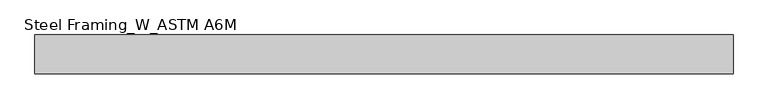
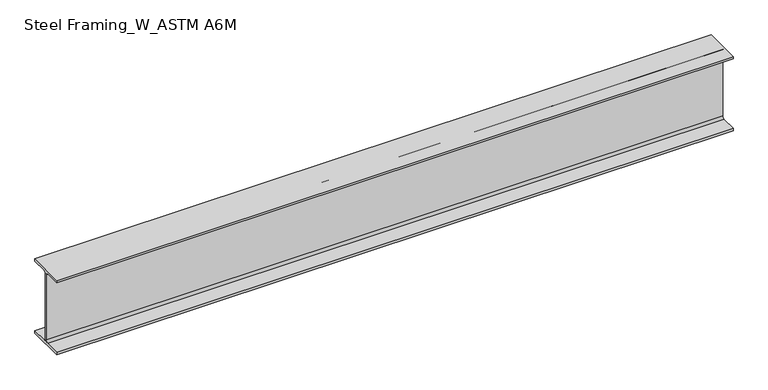
"""IFC4 building model written with IfcOpenShell, lengths in millimetres: beam geometry, Steel Framing_W_ASTM A6M : H_SB_AR_S02_W360x51_G3."""

import ifcopenshell
import ifcopenshell.guid

model = None  # the IFC model being written
_history = None  # IfcOwnerHistory: only IFC2X3 demands one
_inside = {}  # id of a spatial element -> (the spatial element, [elements in it])
_under = {}  # id of a project, library or spatial element -> (it, [spatial elements below it])
_declared = {}  # id of a project -> (the project, [libraries it declares])
_typed = {}  # id of a type object -> (the type object, [elements of that type])
_made_of = {}  # id of a material, layer set ... -> (it, [elements and type objects made of it])


def new_model(schema):
    """Start an empty IFC model of exactly this schema.

    Asked for "IFC4X3", IfcOpenShell would pick the latest addendum, in which some entities
    have other attributes; the version numbers below select the first issue.
    IFC2X3 requires an IfcOwnerHistory on every rooted entity: one is made here for all.
    """
    global model, _history
    if schema == "IFC4X3":
        model = ifcopenshell.file(schema_version=(4, 3, 0, 0))
    else:
        model = ifcopenshell.file(schema=schema)
    _inside.clear()
    _under.clear()
    _declared.clear()
    _typed.clear()
    _made_of.clear()
    _history = None
    if model.schema == "IFC2X3":
        org = make("IfcOrganization", Name="unknown")
        user = make(
            "IfcPersonAndOrganization",
            ThePerson=make("IfcPerson", FamilyName="unknown"),
            TheOrganization=org,
        )
        app = make(
            "IfcApplication",
            ApplicationDeveloper=org,
            Version="unknown",
            ApplicationFullName="unknown",
            ApplicationIdentifier="unknown",
        )
        _history = make(
            "IfcOwnerHistory",
            OwningUser=user,
            OwningApplication=app,
            ChangeAction="ADDED",
            CreationDate=0,
        )
    return model


def make(cls, **values):
    """One entity of the class cls with the attributes given. An attribute that is None is left unset."""
    return model.create_entity(
        cls, **{name: value for name, value in values.items() if value is not None}
    )


def rooted(cls, **values):
    """An entity with a GlobalId (a new one), such as an element, a storey or a relation."""
    return make(cls, GlobalId=ifcopenshell.guid.new(), OwnerHistory=_history, **values)


def si_unit(unit_type, name, prefix=None):
    """IfcSIUnit, for example si_unit("LENGTHUNIT", "METRE", prefix="MILLI")."""
    return make("IfcSIUnit", UnitType=unit_type, Prefix=prefix, Name=name)


def assignment(units):
    """IfcUnitAssignment: the units of a project."""
    return None if units is None else make("IfcUnitAssignment", Units=units)


def point(xyz):
    """IfcCartesianPoint."""
    return None if xyz is None else make("IfcCartesianPoint", Coordinates=xyz)


def direction(xyz):
    """IfcDirection."""
    return None if xyz is None else make("IfcDirection", DirectionRatios=xyz)


def frame(location, z_axis=None, x_axis=None):
    """IfcAxis2Placement3D, a coordinate frame: its origin and axes. An axis left out is left unset."""
    return make(
        "IfcAxis2Placement3D",
        Location=point(location),
        Axis=direction(z_axis),
        RefDirection=direction(x_axis),
    )


def frame_2d(location, x_axis=None):
    """IfcAxis2Placement2D, a coordinate frame in the plane: its origin and x axis."""
    return make(
        "IfcAxis2Placement2D", Location=point(location), RefDirection=direction(x_axis)
    )


def origin():
    """The frame at (0, 0, 0) with its axes left unset."""
    return frame((0.0, 0.0, 0.0))


def place(relative_to, where):
    """IfcLocalPlacement: puts the frame where relative to a parent placement (None: the world)."""
    return make(
        "IfcLocalPlacement", PlacementRelTo=relative_to, RelativePlacement=where
    )


def context(
    kind, dimensions, precision=None, world=None, true_north=None, identifier=None
):
    """IfcGeometricRepresentationContext, for example the 3D "Model" context."""
    return make(
        "IfcGeometricRepresentationContext",
        ContextIdentifier=identifier,
        ContextType=kind,
        CoordinateSpaceDimension=dimensions,
        Precision=precision,
        WorldCoordinateSystem=world,
        TrueNorth=true_north,
    )


def project(units=None, contexts=None):
    """IfcProject with its units and contexts."""
    return rooted(
        "IfcProject",
        Name="project",
        RepresentationContexts=contexts,
        UnitsInContext=assignment(units),
    )


def spatial(cls, under=None, at=None, **own):
    """A site, building, storey or space (cls), placed at a placement, below another one or the project."""
    s = rooted(cls, ObjectPlacement=at, **own)
    if under is not None:
        _under.setdefault(under.id(), (under, []))[1].append(s)
    return s


def polyline(points):
    """IfcPolyline through the points."""
    return make("IfcPolyline", Points=[point(p) for p in points])


def circle_curve(where, radius):
    """IfcCircle in the frame where."""
    return make("IfcCircle", Position=where, Radius=radius)


def trimmed(basis, trim1, trim2, sense, master):
    """IfcTrimmedCurve: the piece of a basis curve between two trims."""
    return make(
        "IfcTrimmedCurve",
        BasisCurve=basis,
        Trim1=trim1,
        Trim2=trim2,
        SenseAgreement=sense,
        MasterRepresentation=master,
    )


def segment(curve, same_sense, transition):
    """IfcCompositeCurveSegment."""
    return make(
        "IfcCompositeCurveSegment",
        Transition=transition,
        SameSense=same_sense,
        ParentCurve=curve,
    )


def composite_curve(segments, self_intersect=None):
    """IfcCompositeCurve: segments joined end to end."""
    return make("IfcCompositeCurve", Segments=segments, SelfIntersect=self_intersect)


def outline(outer, holes=None, kind="AREA"):
    """IfcArbitraryClosedProfileDef: a profile drawn as a closed curve; with holes, ...WithVoids."""
    if holes is None:
        return make("IfcArbitraryClosedProfileDef", ProfileType=kind, OuterCurve=outer)
    return make(
        "IfcArbitraryProfileDefWithVoids",
        ProfileType=kind,
        OuterCurve=outer,
        InnerCurves=holes,
    )


def extrude(swept, where, along, depth):
    """IfcExtrudedAreaSolid: the profile swept, set in the frame where, extruded along a direction by depth."""
    return make(
        "IfcExtrudedAreaSolid",
        SweptArea=swept,
        Position=where,
        ExtrudedDirection=direction(along),
        Depth=depth,
    )


def shape(context_of_items, identifier, shape_type, items):
    """IfcShapeRepresentation: the items that make up one representation, for example the "Body"."""
    return make(
        "IfcShapeRepresentation",
        ContextOfItems=context_of_items,
        RepresentationIdentifier=identifier,
        RepresentationType=shape_type,
        Items=items,
    )


def source(mapping_origin, context_of_items, identifier, shape_type, items):
    """IfcRepresentationMap: a shape defined once, which mapped items show again and again."""
    return make(
        "IfcRepresentationMap",
        MappingOrigin=mapping_origin,
        MappedRepresentation=shape(context_of_items, identifier, shape_type, items),
    )


def transform(
    local_origin,
    x_axis=None,
    y_axis=None,
    z_axis=None,
    scale=None,
    scale2=None,
    scale3=None,
    uniform=True,
):
    """IfcCartesianTransformationOperator3D, or its non-uniform kind. x_axis, y_axis, z_axis: its Axis1, 2, 3."""
    if uniform:
        return make(
            "IfcCartesianTransformationOperator3D",
            Axis1=direction(x_axis),
            Axis2=direction(y_axis),
            LocalOrigin=point(local_origin),
            Scale=scale,
            Axis3=direction(z_axis),
        )
    return make(
        "IfcCartesianTransformationOperator3DnonUniform",
        Axis1=direction(x_axis),
        Axis2=direction(y_axis),
        LocalOrigin=point(local_origin),
        Scale=scale,
        Axis3=direction(z_axis),
        Scale2=scale2,
        Scale3=scale3,
    )


def mapped(mapping_source, mapping_target):
    """IfcMappedItem: shows the shape of a source again, moved by a transform."""
    return make(
        "IfcMappedItem", MappingSource=mapping_source, MappingTarget=mapping_target
    )


def made_of(thing, what):
    """Note that an element or type object is made of a material, layer set ...; save() writes the relation."""
    if what is not None:
        _made_of.setdefault(what.id(), (what, []))[1].append(thing)
    return thing


def element(
    cls,
    number,
    at=None,
    inside=None,
    cuts=None,
    type_object=None,
    material=None,
    context=None,
    identifier="Body",
    shape_type=None,
    held_by="IfcProductDefinitionShape",
    body=None,
    shapes=None,
    **own,
):
    """One element of the class cls, such as IfcWall. Its Tag is "e" and its number.

    at: its placement. inside: the storey or other place that contains it. cuts: it is an
    opening in that element (IfcRelVoidsElement). A single representation is given by context,
    identifier, shape_type and body (its items); several are given by shapes. held_by: the class
    of the entity that holds the representations. save() writes the other relations.
    """
    e = rooted(cls, Tag="e%d" % number, ObjectPlacement=at, **own)
    if body is not None:
        shapes = [shape(context, identifier, shape_type, body)]
    if shapes is not None:
        e.Representation = make(held_by, Representations=shapes)
    if inside is not None:
        _inside.setdefault(inside.id(), (inside, []))[1].append(e)
    if cuts is not None:
        rooted(
            "IfcRelVoidsElement", RelatingBuildingElement=cuts, RelatedOpeningElement=e
        )
    if type_object is not None:
        _typed.setdefault(type_object.id(), (type_object, []))[1].append(e)
    return made_of(e, material)


def aggregate(whole, parts):
    """IfcRelAggregates: a whole, such as a stair, and the parts it consists of."""
    return rooted("IfcRelAggregates", RelatingObject=whole, RelatedObjects=parts)


def save(model, path):
    """Write the relations noted so far, then the file.

    IfcRelAggregates (storeys below a building ...), IfcRelContainedInSpatialStructure (elements
    in a storey), IfcRelDefinesByType, IfcRelAssociatesMaterial and IfcRelDeclares: one each for
    every whole, place, type object, material and project.
    """
    for whole, parts in _under.values():
        aggregate(whole, parts)
    for where, things in _inside.values():
        rooted(
            "IfcRelContainedInSpatialStructure",
            RelatedElements=things,
            RelatingStructure=where,
        )
    for kind, things in _typed.values():
        rooted("IfcRelDefinesByType", RelatedObjects=things, RelatingType=kind)
    for what, things in _made_of.values():
        rooted("IfcRelAssociatesMaterial", RelatedObjects=things, RelatingMaterial=what)
    for by, libraries in _declared.values():
        rooted("IfcRelDeclares", RelatingContext=by, RelatedDefinitions=libraries)
    model.write(path)


def steel_framing_w_astm_a6m_be114a1b(model_context):
    return source(origin(), model_context, "Body", "SweptSolid", [
        extrude(outline(composite_curve([segment(polyline([(85.5, -166.4), (85.5, -178.0), (-85.5, -178.0), (-85.5, -166.4), (-13.72, -166.4)]), True, "CONTINUOUS"), segment(trimmed(circle_curve(frame_2d((-13.72, -156.3)), 10.1), [point((-13.72, -166.4))], [point((-3.62, -156.3))], True, "CARTESIAN"), True, "CONTINUOUS"), segment(polyline([(-3.62, -156.3), (-3.62, 156.3)]), True, "CONTINUOUS"), segment(trimmed(circle_curve(frame_2d((-13.72, 156.3)), 10.1), [point((-3.62, 156.3))], [point((-13.72, 166.4))], True, "CARTESIAN"), True, "CONTINUOUS"), segment(polyline([(-13.72, 166.4), (-85.5, 166.4), (-85.5, 178.0), (85.5, 178.0), (85.5, 166.4), (13.72, 166.4)]), True, "CONTINUOUS"), segment(trimmed(circle_curve(frame_2d((13.72, 156.3)), 10.1), [point((13.72, 166.4))], [point((3.62, 156.3))], True, "CARTESIAN"), True, "CONTINUOUS"), segment(polyline([(3.62, 156.3), (3.62, -156.3)]), True, "CONTINUOUS"), segment(trimmed(circle_curve(frame_2d((13.72, -156.3)), 10.1), [point((3.62, -156.3))], [point((13.72, -166.4))], True, "CARTESIAN"), True, "CONTINUOUS"), segment(polyline([(13.72, -166.4), (85.5, -166.4)]), True, "CONTINUOUS")], self_intersect=False)), frame((-1487.2, 0.0, 0.0), z_axis=(1.0, 0.0, 0.0), x_axis=(0.0, 1.0, 0.0)), (0.0, 0.0, 1.0), 3072.7),
    ])


if __name__ == "__main__":
    model = new_model("IFC4")
    model_context = context("Model", 3, world=origin())
    ifc_project = project(units=[si_unit("LENGTHUNIT", "METRE", prefix="MILLI")], contexts=[model_context])
    site = spatial("IfcSite", under=ifc_project)
    building = spatial("IfcBuilding", under=site)
    placement = place(None, origin())
    steel_framing_w_astm_a6m_shape = steel_framing_w_astm_a6m_be114a1b(model_context)
    element("IfcBeam", 1, ObjectType="Steel Framing_W_ASTM A6M : H_SB_AR_S02_W360x51_G3", at=placement, inside=building, context=model_context, shape_type="MappedRepresentation", body=[
        mapped(steel_framing_w_astm_a6m_shape, transform((0.0, 0.0, 0.0), x_axis=(1.0, 0.0, 0.0), y_axis=(0.0, 1.0, 0.0), z_axis=(0.0, 0.0, 1.0))),
    ])
    save(model, "model.ifc")

# Revit data of these elements
# Type "Steel Framing_W_ASTM A6M : H_SB_AR_S02_W360x51_G3"
#   Type Mark = "G3"
#   Section Name Key = "W14x34"
#   Width = 17.1 cm
#   Web Thickness = 0.724 cm
#   Web Fillet = 1.01 cm
#   Warping Constant = 287000.0 cm⁶
#   Torsional Moment of Inertia = 23.70 cm⁴
#   Section Area = 64.5 cm²
#   Plastic Modulus weak axis = 174.0 cm³
#   Plastic Modulus strong axis = 895.0 cm³
#   Perimeter = 1.36 m²/m
#   Nominal Weight = 51.00 kgf/m
#   Moment of Inertia weak axis = 970.00 cm⁴
#   Moment of Inertia strong axis = 14200.00 cm⁴
#   Height = 35.6 cm
#   Flange Thickness = 1.16 cm
#   Elastic Modulus weak axis = 113.0 cm³
#   Elastic Modulus strong axis = 796.0 cm³
#   Centroid Vertical = 17.8 cm
#   Centroid Horizontal = 8.55 cm
#   Length [instance default] = 1500 mm
#   Structural Material [instance default] = Steel, 45-345
#   Bolt Spacing = 0
#   Assembly Code = ""
# Element 1 (IfcBeam, "Steel Framing_W_ASTM A6M : H_SB_AR_S02_W360x51_G3")
#   Materials on its faces: "Steel, 45-345"
# Materials
#   "Steel, 45-345": class "Metal", colour RGB 189 187 185, transparency 0, Description = "Steel 345 MPa", Cost = 0
